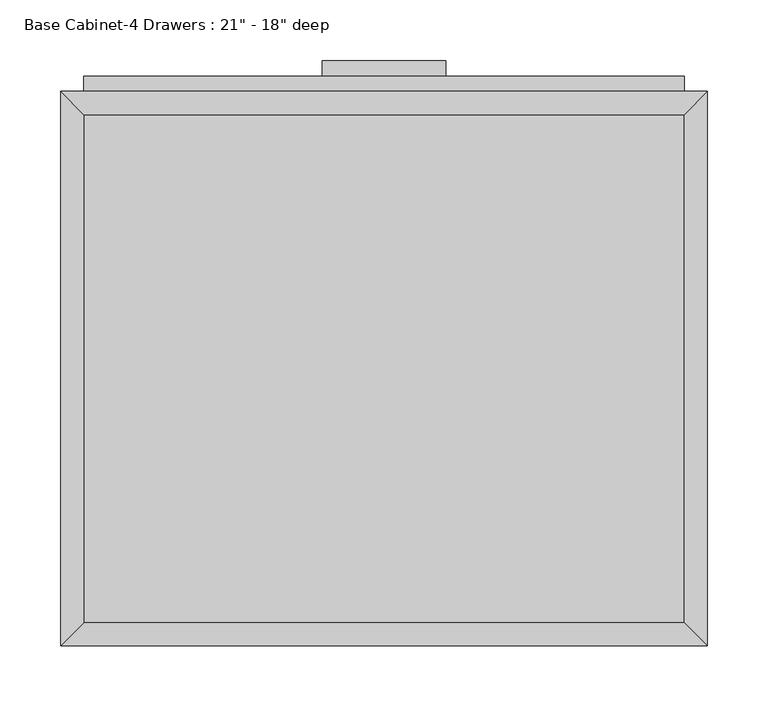
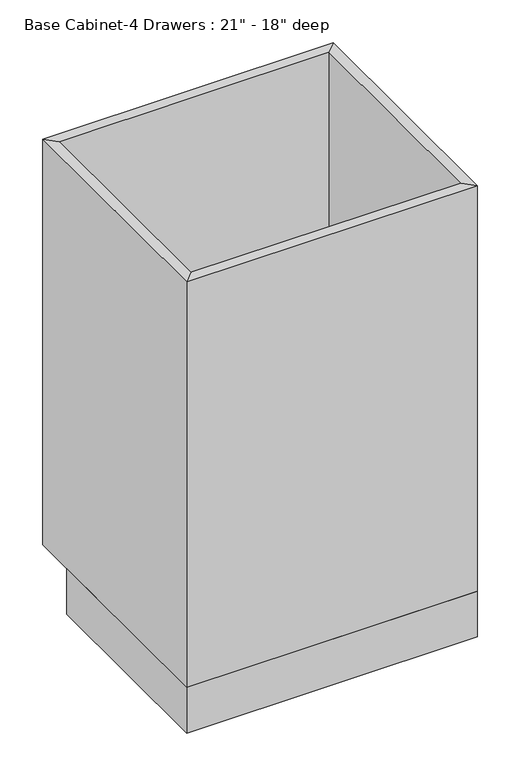
"""IFC4 building model written with IfcOpenShell, lengths in millimetres: furniture geometry."""

from ifc_helpers import new_model, si_unit, frame, origin, origin_with_axes, place, context, project, spatial, polyline, outline, extrude, faceted_brep, source, transform, mapped, element, save


def furniture_352f64ea(model_context):
    return source(origin(), model_context, "Body", "SolidModel", [
        extrude(outline(polyline([(69.5377049, 482.6), (69.5377049, 469.9), (-32.0622951, 469.9), (-32.0622951, 482.6), (69.5377049, 482.6)])), frame((0.0, 0.0, 819.15), z_axis=(0.0, 0.0, 1.0), x_axis=(1.0, 0.0, 0.0)), (0.0, 0.0, 1.0), 12.7),
        extrude(outline(polyline([(69.5377049, 482.6), (69.5377049, 469.9), (-32.0622951, 469.9), (-32.0622951, 482.6), (69.5377049, 482.6)])), frame((0.0, 0.0, 698.5), z_axis=(0.0, 0.0, 1.0), x_axis=(1.0, 0.0, 0.0)), (0.0, 0.0, 1.0), 12.7),
        extrude(outline(polyline([(69.5377049, 482.6), (69.5377049, 469.9), (-32.0622951, 469.9), (-32.0622951, 482.6), (69.5377049, 482.6)])), frame((0.0, 0.0, 546.1), z_axis=(0.0, 0.0, 1.0), x_axis=(1.0, 0.0, 0.0)), (0.0, 0.0, 1.0), 12.7),
        extrude(outline(polyline([(69.5377049, 482.6), (69.5377049, 469.9), (-32.0622951, 469.9), (-32.0622951, 482.6), (69.5377049, 482.6)])), frame((0.0, 0.0, 393.7), z_axis=(0.0, 0.0, 1.0), x_axis=(1.0, 0.0, 0.0)), (0.0, 0.0, 1.0), 12.7),
        extrude(outline(polyline([(266.3877049, 469.9), (266.3877049, 457.2), (-228.9122951, 457.2), (-228.9122951, 469.9), (266.3877049, 469.9)])), frame((0.0, 0.0, 749.3), z_axis=(0.0, 0.0, 1.0), x_axis=(1.0, 0.0, 0.0)), (0.0, 0.0, 1.0), 107.95),
        extrude(outline(polyline([(266.3877049, 469.9), (266.3877049, 457.2), (-228.9122951, 457.2), (-228.9122951, 469.9), (266.3877049, 469.9)])), frame((0.0, 0.0, 596.9), z_axis=(0.0, 0.0, 1.0), x_axis=(1.0, 0.0, 0.0)), (0.0, 0.0, 1.0), 139.7),
        extrude(outline(polyline([(266.3877049, 469.9), (266.3877049, 457.2), (-228.9122951, 457.2), (-228.9122951, 469.9), (266.3877049, 469.9)])), frame((0.0, 0.0, 444.5), z_axis=(0.0, 0.0, 1.0), x_axis=(1.0, 0.0, 0.0)), (0.0, 0.0, 1.0), 139.7),
        extrude(outline(polyline([(266.3877049, 469.9), (266.3877049, 457.2), (-228.9122951, 457.2), (-228.9122951, 469.9), (266.3877049, 469.9)])), frame((0.0, 0.0, 120.65), z_axis=(0.0, 0.0, 1.0), x_axis=(1.0, 0.0, 0.0)), (0.0, 0.0, 1.0), 311.15),
        extrude(outline(polyline([(266.3877049, 19.05), (-228.9122951, 19.05), (-228.9122951, 438.15), (266.3877049, 438.15), (266.3877049, 19.05)])), frame((0.0, 0.0, 88.9), z_axis=(0.0, 0.0, 1.0), x_axis=(1.0, 0.0, 0.0)), (0.0, 0.0, 1.0), 19.05),
        faceted_brep([(266.3877049, 438.15, 876.3), (-228.9122951, 438.15, 876.3), (-228.9122951, 438.15, 88.9), (266.3877049, 438.15, 88.9), (285.4377049, 457.2, 876.3), (-247.9622951, 457.2, 876.3), (285.4377049, 457.2, 88.9), (-247.9622951, 457.2, 88.9), (-228.9122951, 19.05, 876.3), (-228.9122951, 19.05, 88.9), (-247.9622951, 0.0, 876.3), (-247.9622951, 0.0, 88.9), (266.3877049, 19.05, 876.3), (266.3877049, 19.05, 88.9), (285.4377049, 0.0, 876.3), (285.4377049, 0.0, 88.9)], [[[0, 1, 2, 3]], [[4, 5, 1, 0]], [[6, 7, 5, 4]], [[3, 2, 7, 6]], [[1, 8, 9, 2]], [[5, 10, 8, 1]], [[7, 11, 10, 5]], [[2, 9, 11, 7]], [[8, 12, 13, 9]], [[10, 14, 12, 8]], [[11, 15, 14, 10]], [[9, 13, 15, 11]], [[12, 0, 3, 13]], [[14, 4, 0, 12]], [[15, 6, 4, 14]], [[13, 3, 6, 15]]]),
        extrude(outline(polyline([(285.4377049, 0.0), (-247.9622951, 0.0), (-247.9622951, 381.0), (285.4377049, 381.0), (285.4377049, 0.0)])), origin_with_axes(), (0.0, 0.0, 1.0), 88.9),
    ])


if __name__ == "__main__":
    model = new_model("IFC4")
    model_context = context("Model", 3, world=origin())
    ifc_project = project(units=[si_unit("LENGTHUNIT", "METRE", prefix="MILLI")], contexts=[model_context])
    site = spatial("IfcSite", under=ifc_project)
    building = spatial("IfcBuilding", under=site)
    placement = place(None, origin())
    furniture_shape = furniture_352f64ea(model_context)
    element("IfcFurniture", 1, ObjectType="Base Cabinet-4 Drawers : 21\" - 18\" deep", at=placement, inside=building, context=model_context, shape_type="MappedRepresentation", body=[
        mapped(furniture_shape, transform((0.0, 0.0, 0.0), x_axis=(1.0, 0.0, 0.0), y_axis=(0.0, 1.0, 0.0), z_axis=(0.0, 0.0, 1.0))),
    ])
    save(model, "model.ifc")

# Revit data of these elements
# Type "Base Cabinet-4 Drawers : 21\" - 18\" deep"
#   COBie.Type.CreatedBy = "doug.wood@us.ibm.com"
#   COBie.Type.CreatedOn = "2016-04-14T02:07:23"
#   COBie.Type.Name = "Casework_Base Cabinet-4 Drawers_21\" - 18\" deep"
#   COBie.Type.Category = "23-40 35 17 47 11 : Kitchen Casework"
#   COBie.Type.Description = "Base Cabinet-4 Drawers_21\" - 18\" deep"
#   COBie.Type.Manufacturer = ""
#   COBie.Type.ModelNumber = ""
#   Assembly Code = "C1030410"
#   COBie.Type.ReplacementCost = 0
#   Depth = 1' - 6"
#   Height = 2' - 10 1/2"
#   Toe Depth = 0' - 3"
#   Toe Height = 0' - 3 1/2"
#   Width = 1' - 9"
#   COBie.Type = no
#   Cabinet Material = none
#   Door/Drawer Material = none
#   Handle Material = Cabinets - Handles
# Element 1 (IfcFurniture, "Base Cabinet-4 Drawers : 21\" - 18\" deep")
#   Materials on its faces: "Cabinets", "Cabinets - Handles"
# Materials
#   "Cabinets - Handles": class "Metal", colour RGB 57 57 57, transparency 0
#   "Cabinets": class "Miscellaneous", colour RGB 249 249 249, transparency 0
